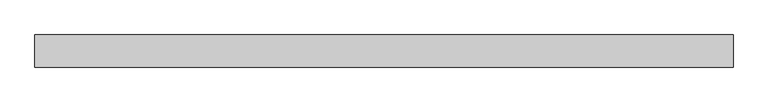
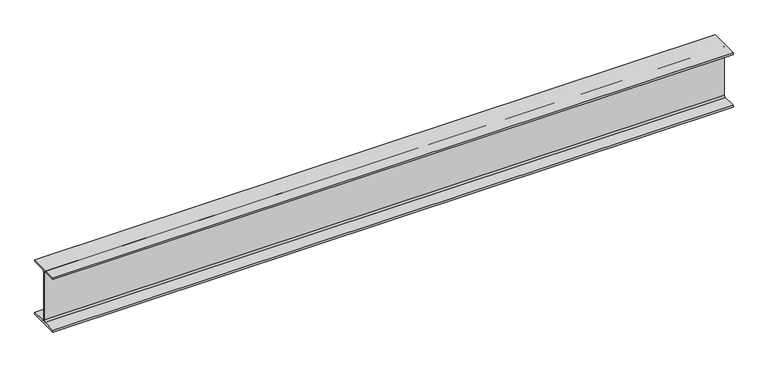
"""IFC4 building model written with IfcOpenShell, lengths in millimetres: beam geometry, Old_Steel Beam_H-KSD3502 : H_SB_ASB_H-200×200x8x12."""

from ifc_helpers import new_model, si_unit, point, frame, frame_2d, origin, place, context, project, spatial, polyline, circle_curve, trimmed, segment, composite_curve, outline, extrude, source, transform, mapped, element, save


def beam_1b7a3572(model_context):
    return source(origin(), model_context, "Body", "SweptSolid", [
        extrude(outline(composite_curve([segment(polyline([(82.5, -141.5), (82.5, -151.7), (-82.5, -151.7), (-82.5, -141.5), (-11.9, -141.5)]), True, "CONTINUOUS"), segment(trimmed(circle_curve(frame_2d((-11.9, -132.6)), 8.9), [point((-11.9, -141.5))], [point((-3.0, -132.6))], True, "CARTESIAN"), True, "CONTINUOUS"), segment(polyline([(-3.0, -132.6), (-3.0, 132.6)]), True, "CONTINUOUS"), segment(trimmed(circle_curve(frame_2d((-11.9, 132.6)), 8.9), [point((-3.0, 132.6))], [point((-11.9, 141.5))], True, "CARTESIAN"), True, "CONTINUOUS"), segment(polyline([(-11.9, 141.5), (-82.5, 141.5), (-82.5, 151.7), (82.5, 151.7), (82.5, 141.5), (11.9, 141.5)]), True, "CONTINUOUS"), segment(trimmed(circle_curve(frame_2d((11.9, 132.6)), 8.9), [point((11.9, 141.5))], [point((3.0, 132.6))], True, "CARTESIAN"), True, "CONTINUOUS"), segment(polyline([(3.0, 132.6), (3.0, -132.6)]), True, "CONTINUOUS"), segment(trimmed(circle_curve(frame_2d((11.9, -132.6)), 8.9), [point((3.0, -132.6))], [point((11.9, -141.5))], True, "CARTESIAN"), True, "CONTINUOUS"), segment(polyline([(11.9, -141.5), (82.5, -141.5)]), True, "CONTINUOUS")], self_intersect=False)), frame((-1654.1298909, 0.0, 0.0), z_axis=(1.0, 0.0, 0.0), x_axis=(0.0, 1.0, 0.0)), (0.0, 0.0, 1.0), 3586.0350237),
    ])


if __name__ == "__main__":
    model = new_model("IFC4")
    model_context = context("Model", 3, world=origin())
    ifc_project = project(units=[si_unit("LENGTHUNIT", "METRE", prefix="MILLI")], contexts=[model_context])
    site = spatial("IfcSite", under=ifc_project)
    building = spatial("IfcBuilding", under=site)
    placement = place(None, origin())
    beam_shape = beam_1b7a3572(model_context)
    element("IfcBeam", 1, ObjectType="Old_Steel Beam_H-KSD3502 : H_SB_ASB_H-200×200x8x12", at=placement, inside=building, context=model_context, shape_type="MappedRepresentation", body=[
        mapped(beam_shape, transform((0.0, 0.0, 0.0), x_axis=(1.0, 0.0, 0.0), y_axis=(0.0, 1.0, 0.0), z_axis=(0.0, 0.0, 1.0))),
    ])
    save(model, "model.ifc")

# Revit data of these elements
# Type "Old_Steel Beam_H-KSD3502 : H_SB_ASB_H-200×200x8x12"
#   Width = 20.0 cm
#   Web Thickness = 0.8 cm
#   Web Fillet = 1.3 cm
#   Warping Constant = 141376.0 cm⁶
#   Torsional Moment of Inertia = 26.2485 cm⁴
#   Torsional Modulus = 1.0 cm³
#   Section Area = 63.53 cm²
#   Plastic Modulus weak axis = 244.0 cm³
#   Plastic Modulus strong axis = 525.0 cm³
#   Perimeter = 1.16 m²/m
#   Nominal Weight = 49.90 kgf/m
#   Moment of Inertia weak axis = 1600.00 cm⁴
#   Moment of Inertia strong axis = 4720.00 cm⁴
#   Height = 20.0 cm
#   Flange Thickness = 1.2 cm
#   Elastic Modulus weak axis = 160.0 cm³
#   Elastic Modulus strong axis = 472.0 cm³
#   Centroid Vertical = 10.0 cm
#   Centroid Horizontal = 10.0 cm
#   Length [instance default] = 1.5240 m
#   Structural Material [instance default] = Steel, 45-345
#   Assembly Code = ""
# Element 1 (IfcBeam, "Old_Steel Beam_H-KSD3502 : H_SB_ASB_H-200×200x8x12")
#   Structural Material = none
# Materials
#   "Steel, 45-345": class "Metal", colour RGB 189 187 185, transparency 0, Description = "Steel 345 MPa", Cost = 0
